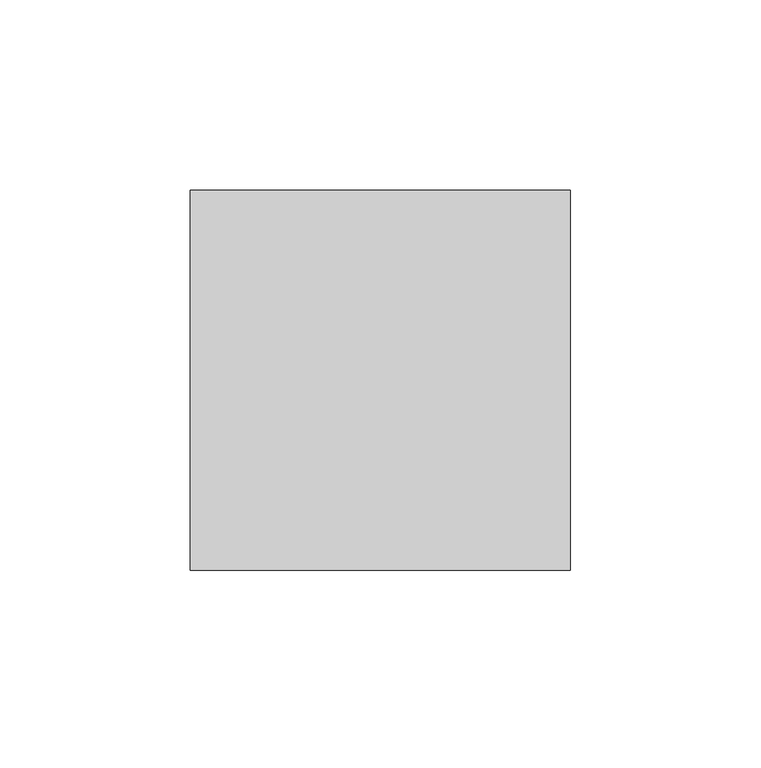
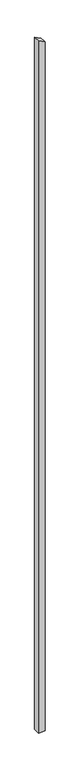
"""IFC4 building model written with IfcOpenShell, lengths in millimetres: column geometry, Holzstütze 158706 : Holzstütze 158706."""

import ifcopenshell
import ifcopenshell.guid

model = None  # the IFC model being written
_history = None  # IfcOwnerHistory: only IFC2X3 demands one
_inside = {}  # id of a spatial element -> (the spatial element, [elements in it])
_under = {}  # id of a project, library or spatial element -> (it, [spatial elements below it])
_declared = {}  # id of a project -> (the project, [libraries it declares])
_typed = {}  # id of a type object -> (the type object, [elements of that type])
_made_of = {}  # id of a material, layer set ... -> (it, [elements and type objects made of it])


def new_model(schema):
    """Start an empty IFC model of exactly this schema.

    Asked for "IFC4X3", IfcOpenShell would pick the latest addendum, in which some entities
    have other attributes; the version numbers below select the first issue.
    IFC2X3 requires an IfcOwnerHistory on every rooted entity: one is made here for all.
    """
    global model, _history
    if schema == "IFC4X3":
        model = ifcopenshell.file(schema_version=(4, 3, 0, 0))
    else:
        model = ifcopenshell.file(schema=schema)
    _inside.clear()
    _under.clear()
    _declared.clear()
    _typed.clear()
    _made_of.clear()
    _history = None
    if model.schema == "IFC2X3":
        org = make("IfcOrganization", Name="unknown")
        user = make(
            "IfcPersonAndOrganization",
            ThePerson=make("IfcPerson", FamilyName="unknown"),
            TheOrganization=org,
        )
        app = make(
            "IfcApplication",
            ApplicationDeveloper=org,
            Version="unknown",
            ApplicationFullName="unknown",
            ApplicationIdentifier="unknown",
        )
        _history = make(
            "IfcOwnerHistory",
            OwningUser=user,
            OwningApplication=app,
            ChangeAction="ADDED",
            CreationDate=0,
        )
    return model


def make(cls, **values):
    """One entity of the class cls with the attributes given. An attribute that is None is left unset."""
    return model.create_entity(
        cls, **{name: value for name, value in values.items() if value is not None}
    )


def rooted(cls, **values):
    """An entity with a GlobalId (a new one), such as an element, a storey or a relation."""
    return make(cls, GlobalId=ifcopenshell.guid.new(), OwnerHistory=_history, **values)


def si_unit(unit_type, name, prefix=None):
    """IfcSIUnit, for example si_unit("LENGTHUNIT", "METRE", prefix="MILLI")."""
    return make("IfcSIUnit", UnitType=unit_type, Prefix=prefix, Name=name)


def assignment(units):
    """IfcUnitAssignment: the units of a project."""
    return None if units is None else make("IfcUnitAssignment", Units=units)


def point(xyz):
    """IfcCartesianPoint."""
    return None if xyz is None else make("IfcCartesianPoint", Coordinates=xyz)


def direction(xyz):
    """IfcDirection."""
    return None if xyz is None else make("IfcDirection", DirectionRatios=xyz)


def frame(location, z_axis=None, x_axis=None):
    """IfcAxis2Placement3D, a coordinate frame: its origin and axes. An axis left out is left unset."""
    return make(
        "IfcAxis2Placement3D",
        Location=point(location),
        Axis=direction(z_axis),
        RefDirection=direction(x_axis),
    )


def origin():
    """The frame at (0, 0, 0) with its axes left unset."""
    return frame((0.0, 0.0, 0.0))


def place(relative_to, where):
    """IfcLocalPlacement: puts the frame where relative to a parent placement (None: the world)."""
    return make(
        "IfcLocalPlacement", PlacementRelTo=relative_to, RelativePlacement=where
    )


def context(
    kind, dimensions, precision=None, world=None, true_north=None, identifier=None
):
    """IfcGeometricRepresentationContext, for example the 3D "Model" context."""
    return make(
        "IfcGeometricRepresentationContext",
        ContextIdentifier=identifier,
        ContextType=kind,
        CoordinateSpaceDimension=dimensions,
        Precision=precision,
        WorldCoordinateSystem=world,
        TrueNorth=true_north,
    )


def project(units=None, contexts=None):
    """IfcProject with its units and contexts."""
    return rooted(
        "IfcProject",
        Name="project",
        RepresentationContexts=contexts,
        UnitsInContext=assignment(units),
    )


def spatial(cls, under=None, at=None, **own):
    """A site, building, storey or space (cls), placed at a placement, below another one or the project."""
    s = rooted(cls, ObjectPlacement=at, **own)
    if under is not None:
        _under.setdefault(under.id(), (under, []))[1].append(s)
    return s


def polyline(points):
    """IfcPolyline through the points."""
    return make("IfcPolyline", Points=[point(p) for p in points])


def outline(outer, holes=None, kind="AREA"):
    """IfcArbitraryClosedProfileDef: a profile drawn as a closed curve; with holes, ...WithVoids."""
    if holes is None:
        return make("IfcArbitraryClosedProfileDef", ProfileType=kind, OuterCurve=outer)
    return make(
        "IfcArbitraryProfileDefWithVoids",
        ProfileType=kind,
        OuterCurve=outer,
        InnerCurves=holes,
    )


def extrude(swept, where, along, depth):
    """IfcExtrudedAreaSolid: the profile swept, set in the frame where, extruded along a direction by depth."""
    return make(
        "IfcExtrudedAreaSolid",
        SweptArea=swept,
        Position=where,
        ExtrudedDirection=direction(along),
        Depth=depth,
    )


def shape(context_of_items, identifier, shape_type, items):
    """IfcShapeRepresentation: the items that make up one representation, for example the "Body"."""
    return make(
        "IfcShapeRepresentation",
        ContextOfItems=context_of_items,
        RepresentationIdentifier=identifier,
        RepresentationType=shape_type,
        Items=items,
    )


def source(mapping_origin, context_of_items, identifier, shape_type, items):
    """IfcRepresentationMap: a shape defined once, which mapped items show again and again."""
    return make(
        "IfcRepresentationMap",
        MappingOrigin=mapping_origin,
        MappedRepresentation=shape(context_of_items, identifier, shape_type, items),
    )


def transform(
    local_origin,
    x_axis=None,
    y_axis=None,
    z_axis=None,
    scale=None,
    scale2=None,
    scale3=None,
    uniform=True,
):
    """IfcCartesianTransformationOperator3D, or its non-uniform kind. x_axis, y_axis, z_axis: its Axis1, 2, 3."""
    if uniform:
        return make(
            "IfcCartesianTransformationOperator3D",
            Axis1=direction(x_axis),
            Axis2=direction(y_axis),
            LocalOrigin=point(local_origin),
            Scale=scale,
            Axis3=direction(z_axis),
        )
    return make(
        "IfcCartesianTransformationOperator3DnonUniform",
        Axis1=direction(x_axis),
        Axis2=direction(y_axis),
        LocalOrigin=point(local_origin),
        Scale=scale,
        Axis3=direction(z_axis),
        Scale2=scale2,
        Scale3=scale3,
    )


def mapped(mapping_source, mapping_target):
    """IfcMappedItem: shows the shape of a source again, moved by a transform."""
    return make(
        "IfcMappedItem", MappingSource=mapping_source, MappingTarget=mapping_target
    )


def made_of(thing, what):
    """Note that an element or type object is made of a material, layer set ...; save() writes the relation."""
    if what is not None:
        _made_of.setdefault(what.id(), (what, []))[1].append(thing)
    return thing


def element(
    cls,
    number,
    at=None,
    inside=None,
    cuts=None,
    type_object=None,
    material=None,
    context=None,
    identifier="Body",
    shape_type=None,
    held_by="IfcProductDefinitionShape",
    body=None,
    shapes=None,
    **own,
):
    """One element of the class cls, such as IfcWall. Its Tag is "e" and its number.

    at: its placement. inside: the storey or other place that contains it. cuts: it is an
    opening in that element (IfcRelVoidsElement). A single representation is given by context,
    identifier, shape_type and body (its items); several are given by shapes. held_by: the class
    of the entity that holds the representations. save() writes the other relations.
    """
    e = rooted(cls, Tag="e%d" % number, ObjectPlacement=at, **own)
    if body is not None:
        shapes = [shape(context, identifier, shape_type, body)]
    if shapes is not None:
        e.Representation = make(held_by, Representations=shapes)
    if inside is not None:
        _inside.setdefault(inside.id(), (inside, []))[1].append(e)
    if cuts is not None:
        rooted(
            "IfcRelVoidsElement", RelatingBuildingElement=cuts, RelatedOpeningElement=e
        )
    if type_object is not None:
        _typed.setdefault(type_object.id(), (type_object, []))[1].append(e)
    return made_of(e, material)


def aggregate(whole, parts):
    """IfcRelAggregates: a whole, such as a stair, and the parts it consists of."""
    return rooted("IfcRelAggregates", RelatingObject=whole, RelatedObjects=parts)


def save(model, path):
    """Write the relations noted so far, then the file.

    IfcRelAggregates (storeys below a building ...), IfcRelContainedInSpatialStructure (elements
    in a storey), IfcRelDefinesByType, IfcRelAssociatesMaterial and IfcRelDeclares: one each for
    every whole, place, type object, material and project.
    """
    for whole, parts in _under.values():
        aggregate(whole, parts)
    for where, things in _inside.values():
        rooted(
            "IfcRelContainedInSpatialStructure",
            RelatedElements=things,
            RelatingStructure=where,
        )
    for kind, things in _typed.values():
        rooted("IfcRelDefinesByType", RelatedObjects=things, RelatingType=kind)
    for what, things in _made_of.values():
        rooted("IfcRelAssociatesMaterial", RelatedObjects=things, RelatingMaterial=what)
    for by, libraries in _declared.values():
        rooted("IfcRelDeclares", RelatingContext=by, RelatedDefinitions=libraries)
    model.write(path)


def column_2f8b9505(model_context):
    return source(origin(), model_context, "Body", "SweptSolid", [
        extrude(outline(polyline([(-500.0, 165867.7593015), (-500.0, 165967.7593015), (10590.0588201, 165967.7593015), (10641.011365, 165867.7593015), (-500.0, 165867.7593015)])), frame((0.0, 47884.7962965, 0.0), z_axis=(0.0, 1.0, 0.0), x_axis=(0.0, 0.0, 1.0)), (0.0, 0.0, 1.0), 100.0),
    ])


if __name__ == "__main__":
    model = new_model("IFC4")
    model_context = context("Model", 3, world=origin())
    ifc_project = project(units=[si_unit("LENGTHUNIT", "METRE", prefix="MILLI")], contexts=[model_context])
    site = spatial("IfcSite", under=ifc_project)
    building = spatial("IfcBuilding", under=site)
    placement = place(None, origin())
    column_shape = column_2f8b9505(model_context)
    element("IfcColumn", 1, ObjectType="Holzstütze 158706 : Holzstütze 158706", at=placement, inside=building, context=model_context, shape_type="MappedRepresentation", body=[
        mapped(column_shape, transform((0.0, 0.0, 0.0), x_axis=(1.0, 0.0, 0.0), y_axis=(0.0, 1.0, 0.0), z_axis=(0.0, 0.0, 1.0))),
    ])
    save(model, "model.ifc")

# Revit data of these elements
# Project information
#   Organization Name = "Organization Name"
#   Organization Description = "Organization Description"
#   Building Name = "Building Name"
#   IfcOrganization = "KURIARCHITEKTEN"
#   IfcApplicationVersion = "2023.1"
#   IfcApplicationName = "Allplan"
#   IfcSite GUID = "3xMs$kp1n46ejeur8tozco"
#   IfcBuilding GUID = "0i8UyhEYT3nv9HLlo1H2X7"
#   IfcProject GUID = "2x1YFttxr4OvBiL8xtaqeA"
#   NameOverride = "GEBÄUDE 1"
#   Project Issue Date = "Issue Date"
#   Project Status = "Project Status"
#   Client Name = "Client Name"
#   Project Address = "Enter address here\nAddress Line 2"
#   Project Name = "Project Name"
#   Project Number = "Project Number"
# Type "Holzstütze 158706 : Holzstütze 158706"
#   Abrechnungsart = "m"
#   Allright_Bauteil_ID = "0152St 0000143525"
#   Bezeichnung = "Holzstütze"
#   Codetext = "ST-HOLZ\\"
#   Gewerk = "Zimmer- und Holzbauarbeiten"
#   Material = "Holz"
#   Objektname = "Stütze"
#   NameOverride = "Holzstütze"
#   Reference = "Holzstütze"
#   Status = "NEW"
#   ThermalTransmittance = 0.0000 BTU/(h·ft²·°F)
#   Roll = 0.00°
#   Slope = 0.00°
#   2D Interaktion = yes
#   IsExternal = yes
#   LoadBearing = yes
# Element 1 (IfcColumn, "Holzstütze 158706 : Holzstütze 158706")
#   Materials on its faces: "holzschalung"
# Materials
#   "holzschalung": class "Unassigned", colour RGB 128 128 128, transparency 0
